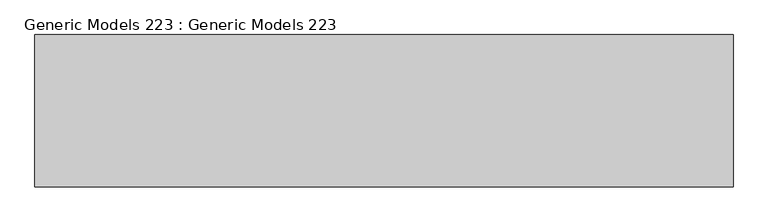
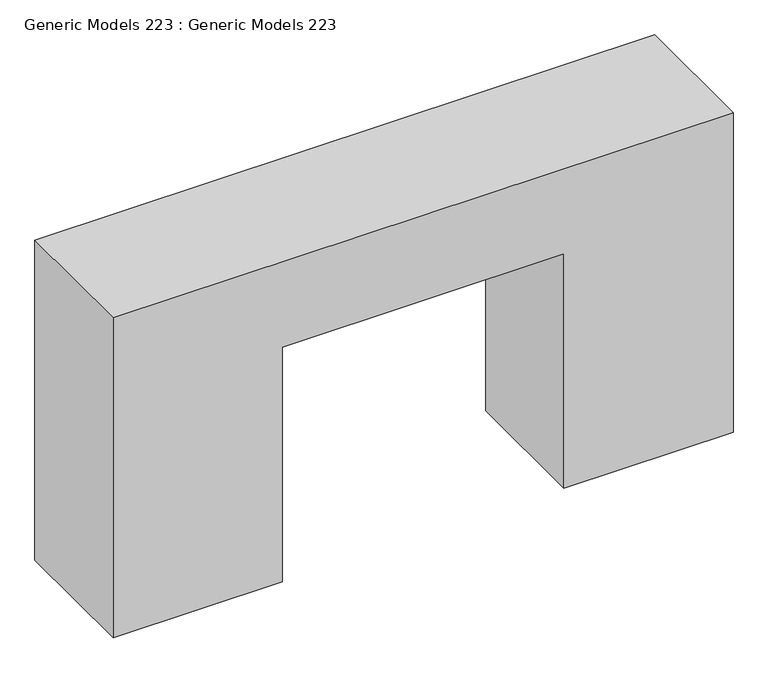
"""IFC4 building model written with IfcOpenShell, lengths in millimetres: proxy geometry, Generic Models 223 : Generic Models 223."""

import ifcopenshell
import ifcopenshell.guid

model = None  # the IFC model being written
_history = None  # IfcOwnerHistory: only IFC2X3 demands one
_inside = {}  # id of a spatial element -> (the spatial element, [elements in it])
_under = {}  # id of a project, library or spatial element -> (it, [spatial elements below it])
_declared = {}  # id of a project -> (the project, [libraries it declares])
_typed = {}  # id of a type object -> (the type object, [elements of that type])
_made_of = {}  # id of a material, layer set ... -> (it, [elements and type objects made of it])


def new_model(schema):
    """Start an empty IFC model of exactly this schema.

    Asked for "IFC4X3", IfcOpenShell would pick the latest addendum, in which some entities
    have other attributes; the version numbers below select the first issue.
    IFC2X3 requires an IfcOwnerHistory on every rooted entity: one is made here for all.
    """
    global model, _history
    if schema == "IFC4X3":
        model = ifcopenshell.file(schema_version=(4, 3, 0, 0))
    else:
        model = ifcopenshell.file(schema=schema)
    _inside.clear()
    _under.clear()
    _declared.clear()
    _typed.clear()
    _made_of.clear()
    _history = None
    if model.schema == "IFC2X3":
        org = make("IfcOrganization", Name="unknown")
        user = make(
            "IfcPersonAndOrganization",
            ThePerson=make("IfcPerson", FamilyName="unknown"),
            TheOrganization=org,
        )
        app = make(
            "IfcApplication",
            ApplicationDeveloper=org,
            Version="unknown",
            ApplicationFullName="unknown",
            ApplicationIdentifier="unknown",
        )
        _history = make(
            "IfcOwnerHistory",
            OwningUser=user,
            OwningApplication=app,
            ChangeAction="ADDED",
            CreationDate=0,
        )
    return model


def make(cls, **values):
    """One entity of the class cls with the attributes given. An attribute that is None is left unset."""
    return model.create_entity(
        cls, **{name: value for name, value in values.items() if value is not None}
    )


def rooted(cls, **values):
    """An entity with a GlobalId (a new one), such as an element, a storey or a relation."""
    return make(cls, GlobalId=ifcopenshell.guid.new(), OwnerHistory=_history, **values)


def si_unit(unit_type, name, prefix=None):
    """IfcSIUnit, for example si_unit("LENGTHUNIT", "METRE", prefix="MILLI")."""
    return make("IfcSIUnit", UnitType=unit_type, Prefix=prefix, Name=name)


def assignment(units):
    """IfcUnitAssignment: the units of a project."""
    return None if units is None else make("IfcUnitAssignment", Units=units)


def point(xyz):
    """IfcCartesianPoint."""
    return None if xyz is None else make("IfcCartesianPoint", Coordinates=xyz)


def direction(xyz):
    """IfcDirection."""
    return None if xyz is None else make("IfcDirection", DirectionRatios=xyz)


def frame(location, z_axis=None, x_axis=None):
    """IfcAxis2Placement3D, a coordinate frame: its origin and axes. An axis left out is left unset."""
    return make(
        "IfcAxis2Placement3D",
        Location=point(location),
        Axis=direction(z_axis),
        RefDirection=direction(x_axis),
    )


def origin():
    """The frame at (0, 0, 0) with its axes left unset."""
    return frame((0.0, 0.0, 0.0))


def place(relative_to, where):
    """IfcLocalPlacement: puts the frame where relative to a parent placement (None: the world)."""
    return make(
        "IfcLocalPlacement", PlacementRelTo=relative_to, RelativePlacement=where
    )


def context(
    kind, dimensions, precision=None, world=None, true_north=None, identifier=None
):
    """IfcGeometricRepresentationContext, for example the 3D "Model" context."""
    return make(
        "IfcGeometricRepresentationContext",
        ContextIdentifier=identifier,
        ContextType=kind,
        CoordinateSpaceDimension=dimensions,
        Precision=precision,
        WorldCoordinateSystem=world,
        TrueNorth=true_north,
    )


def project(units=None, contexts=None):
    """IfcProject with its units and contexts."""
    return rooted(
        "IfcProject",
        Name="project",
        RepresentationContexts=contexts,
        UnitsInContext=assignment(units),
    )


def spatial(cls, under=None, at=None, **own):
    """A site, building, storey or space (cls), placed at a placement, below another one or the project."""
    s = rooted(cls, ObjectPlacement=at, **own)
    if under is not None:
        _under.setdefault(under.id(), (under, []))[1].append(s)
    return s


def polyline(points):
    """IfcPolyline through the points."""
    return make("IfcPolyline", Points=[point(p) for p in points])


def outline(outer, holes=None, kind="AREA"):
    """IfcArbitraryClosedProfileDef: a profile drawn as a closed curve; with holes, ...WithVoids."""
    if holes is None:
        return make("IfcArbitraryClosedProfileDef", ProfileType=kind, OuterCurve=outer)
    return make(
        "IfcArbitraryProfileDefWithVoids",
        ProfileType=kind,
        OuterCurve=outer,
        InnerCurves=holes,
    )


def extrude(swept, where, along, depth):
    """IfcExtrudedAreaSolid: the profile swept, set in the frame where, extruded along a direction by depth."""
    return make(
        "IfcExtrudedAreaSolid",
        SweptArea=swept,
        Position=where,
        ExtrudedDirection=direction(along),
        Depth=depth,
    )


def shape(context_of_items, identifier, shape_type, items):
    """IfcShapeRepresentation: the items that make up one representation, for example the "Body"."""
    return make(
        "IfcShapeRepresentation",
        ContextOfItems=context_of_items,
        RepresentationIdentifier=identifier,
        RepresentationType=shape_type,
        Items=items,
    )


def source(mapping_origin, context_of_items, identifier, shape_type, items):
    """IfcRepresentationMap: a shape defined once, which mapped items show again and again."""
    return make(
        "IfcRepresentationMap",
        MappingOrigin=mapping_origin,
        MappedRepresentation=shape(context_of_items, identifier, shape_type, items),
    )


def transform(
    local_origin,
    x_axis=None,
    y_axis=None,
    z_axis=None,
    scale=None,
    scale2=None,
    scale3=None,
    uniform=True,
):
    """IfcCartesianTransformationOperator3D, or its non-uniform kind. x_axis, y_axis, z_axis: its Axis1, 2, 3."""
    if uniform:
        return make(
            "IfcCartesianTransformationOperator3D",
            Axis1=direction(x_axis),
            Axis2=direction(y_axis),
            LocalOrigin=point(local_origin),
            Scale=scale,
            Axis3=direction(z_axis),
        )
    return make(
        "IfcCartesianTransformationOperator3DnonUniform",
        Axis1=direction(x_axis),
        Axis2=direction(y_axis),
        LocalOrigin=point(local_origin),
        Scale=scale,
        Axis3=direction(z_axis),
        Scale2=scale2,
        Scale3=scale3,
    )


def mapped(mapping_source, mapping_target):
    """IfcMappedItem: shows the shape of a source again, moved by a transform."""
    return make(
        "IfcMappedItem", MappingSource=mapping_source, MappingTarget=mapping_target
    )


def made_of(thing, what):
    """Note that an element or type object is made of a material, layer set ...; save() writes the relation."""
    if what is not None:
        _made_of.setdefault(what.id(), (what, []))[1].append(thing)
    return thing


def element(
    cls,
    number,
    at=None,
    inside=None,
    cuts=None,
    type_object=None,
    material=None,
    context=None,
    identifier="Body",
    shape_type=None,
    held_by="IfcProductDefinitionShape",
    body=None,
    shapes=None,
    **own,
):
    """One element of the class cls, such as IfcWall. Its Tag is "e" and its number.

    at: its placement. inside: the storey or other place that contains it. cuts: it is an
    opening in that element (IfcRelVoidsElement). A single representation is given by context,
    identifier, shape_type and body (its items); several are given by shapes. held_by: the class
    of the entity that holds the representations. save() writes the other relations.
    """
    e = rooted(cls, Tag="e%d" % number, ObjectPlacement=at, **own)
    if body is not None:
        shapes = [shape(context, identifier, shape_type, body)]
    if shapes is not None:
        e.Representation = make(held_by, Representations=shapes)
    if inside is not None:
        _inside.setdefault(inside.id(), (inside, []))[1].append(e)
    if cuts is not None:
        rooted(
            "IfcRelVoidsElement", RelatingBuildingElement=cuts, RelatedOpeningElement=e
        )
    if type_object is not None:
        _typed.setdefault(type_object.id(), (type_object, []))[1].append(e)
    return made_of(e, material)


def aggregate(whole, parts):
    """IfcRelAggregates: a whole, such as a stair, and the parts it consists of."""
    return rooted("IfcRelAggregates", RelatingObject=whole, RelatedObjects=parts)


def save(model, path):
    """Write the relations noted so far, then the file.

    IfcRelAggregates (storeys below a building ...), IfcRelContainedInSpatialStructure (elements
    in a storey), IfcRelDefinesByType, IfcRelAssociatesMaterial and IfcRelDeclares: one each for
    every whole, place, type object, material and project.
    """
    for whole, parts in _under.values():
        aggregate(whole, parts)
    for where, things in _inside.values():
        rooted(
            "IfcRelContainedInSpatialStructure",
            RelatedElements=things,
            RelatingStructure=where,
        )
    for kind, things in _typed.values():
        rooted("IfcRelDefinesByType", RelatedObjects=things, RelatingType=kind)
    for what, things in _made_of.values():
        rooted("IfcRelAssociatesMaterial", RelatedObjects=things, RelatingMaterial=what)
    for by, libraries in _declared.values():
        rooted("IfcRelDeclares", RelatingContext=by, RelatedDefinitions=libraries)
    model.write(path)


def generic_models_223_generic_models_223_4d8b3dd8(model_context):
    return source(origin(), model_context, "Body", "SweptSolid", [
        extrude(outline(polyline([(123754.896, 8572.3263705), (123754.896, 7175.3263704), (122992.896, 7175.3263704), (122992.896, 7556.3263704), (123551.696, 7556.3263704), (123551.696, 8191.3263705), (122992.896, 8191.3263705), (122992.896, 8572.3263705), (123754.896, 8572.3263705)])), frame((0.0, 4260.0872686, 0.0), z_axis=(0.0, 1.0, 0.0), x_axis=(0.0, 0.0, 1.0)), (0.0, 0.0, 1.0), 304.8),
    ])


if __name__ == "__main__":
    model = new_model("IFC4")
    model_context = context("Model", 3, world=origin())
    ifc_project = project(units=[si_unit("LENGTHUNIT", "METRE", prefix="MILLI")], contexts=[model_context])
    site = spatial("IfcSite", under=ifc_project)
    building = spatial("IfcBuilding", under=site)
    placement = place(None, origin())
    generic_models_223_generic_models_223_shape = generic_models_223_generic_models_223_4d8b3dd8(model_context)
    element("IfcBuildingElementProxy", 1, Name="Generic Models 223 : Generic Models 223", ObjectType="Generic Models 223 : Generic Models 223", at=placement, inside=building, context=model_context, shape_type="MappedRepresentation", body=[
        mapped(generic_models_223_generic_models_223_shape, transform((0.0, 0.0, 0.0), x_axis=(1.0, 0.0, 0.0), y_axis=(0.0, 1.0, 0.0), z_axis=(0.0, 0.0, 1.0))),
    ])
    save(model, "model.ifc")

# Revit data of these elements
# Element 1 (IfcBuildingElementProxy, "Generic Models 223 : Generic Models 223")
#   Materials on its faces: "_CONCRETE SLAB W/ WIRE MESH (SEE STRUCT. DWGS)"
# Materials
#   "_CONCRETE SLAB W/ WIRE MESH (SEE STRUCT. DWGS)": class "Generic", colour RGB 191 191 191, transparency 0, Cost = 0
